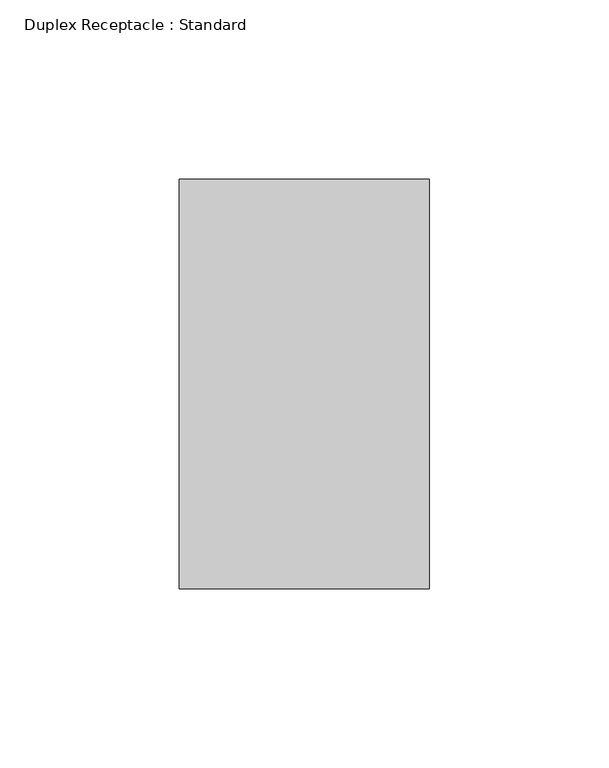
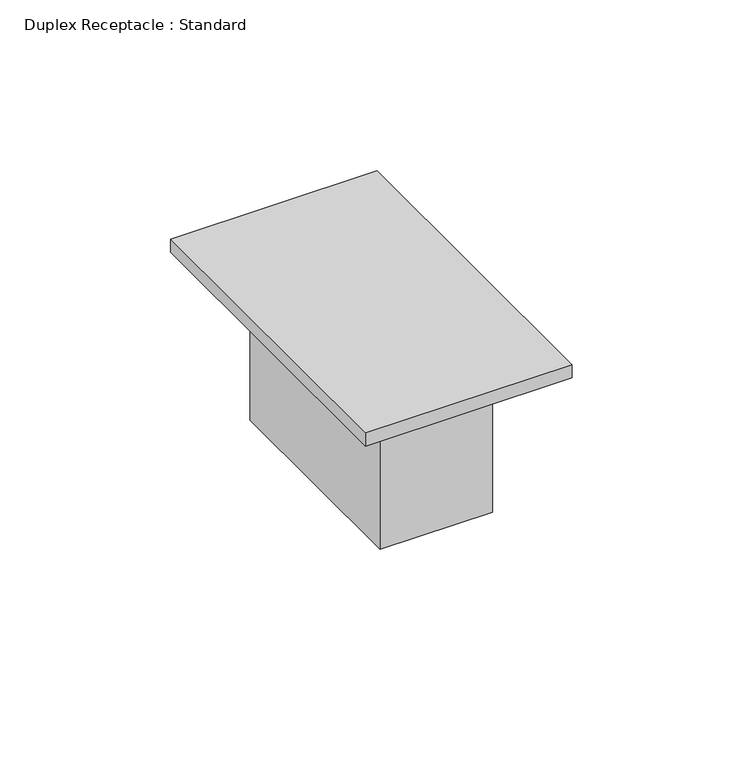
"""IFC4 building model written with IfcOpenShell, lengths in millimetres: proxy geometry, Duplex Receptacle : Standard."""

import ifcopenshell
import ifcopenshell.guid

model = None  # the IFC model being written
_history = None  # IfcOwnerHistory: only IFC2X3 demands one
_inside = {}  # id of a spatial element -> (the spatial element, [elements in it])
_under = {}  # id of a project, library or spatial element -> (it, [spatial elements below it])
_declared = {}  # id of a project -> (the project, [libraries it declares])
_typed = {}  # id of a type object -> (the type object, [elements of that type])
_made_of = {}  # id of a material, layer set ... -> (it, [elements and type objects made of it])


def new_model(schema):
    """Start an empty IFC model of exactly this schema.

    Asked for "IFC4X3", IfcOpenShell would pick the latest addendum, in which some entities
    have other attributes; the version numbers below select the first issue.
    IFC2X3 requires an IfcOwnerHistory on every rooted entity: one is made here for all.
    """
    global model, _history
    if schema == "IFC4X3":
        model = ifcopenshell.file(schema_version=(4, 3, 0, 0))
    else:
        model = ifcopenshell.file(schema=schema)
    _inside.clear()
    _under.clear()
    _declared.clear()
    _typed.clear()
    _made_of.clear()
    _history = None
    if model.schema == "IFC2X3":
        org = make("IfcOrganization", Name="unknown")
        user = make(
            "IfcPersonAndOrganization",
            ThePerson=make("IfcPerson", FamilyName="unknown"),
            TheOrganization=org,
        )
        app = make(
            "IfcApplication",
            ApplicationDeveloper=org,
            Version="unknown",
            ApplicationFullName="unknown",
            ApplicationIdentifier="unknown",
        )
        _history = make(
            "IfcOwnerHistory",
            OwningUser=user,
            OwningApplication=app,
            ChangeAction="ADDED",
            CreationDate=0,
        )
    return model


def make(cls, **values):
    """One entity of the class cls with the attributes given. An attribute that is None is left unset."""
    return model.create_entity(
        cls, **{name: value for name, value in values.items() if value is not None}
    )


def rooted(cls, **values):
    """An entity with a GlobalId (a new one), such as an element, a storey or a relation."""
    return make(cls, GlobalId=ifcopenshell.guid.new(), OwnerHistory=_history, **values)


def si_unit(unit_type, name, prefix=None):
    """IfcSIUnit, for example si_unit("LENGTHUNIT", "METRE", prefix="MILLI")."""
    return make("IfcSIUnit", UnitType=unit_type, Prefix=prefix, Name=name)


def assignment(units):
    """IfcUnitAssignment: the units of a project."""
    return None if units is None else make("IfcUnitAssignment", Units=units)


def point(xyz):
    """IfcCartesianPoint."""
    return None if xyz is None else make("IfcCartesianPoint", Coordinates=xyz)


def direction(xyz):
    """IfcDirection."""
    return None if xyz is None else make("IfcDirection", DirectionRatios=xyz)


def frame(location, z_axis=None, x_axis=None):
    """IfcAxis2Placement3D, a coordinate frame: its origin and axes. An axis left out is left unset."""
    return make(
        "IfcAxis2Placement3D",
        Location=point(location),
        Axis=direction(z_axis),
        RefDirection=direction(x_axis),
    )


def origin():
    """The frame at (0, 0, 0) with its axes left unset."""
    return frame((0.0, 0.0, 0.0))


def origin_with_axes():
    """The frame at (0, 0, 0) with the z axis (0, 0, 1) and the x axis (1, 0, 0) written out."""
    return frame((0.0, 0.0, 0.0), z_axis=(0.0, 0.0, 1.0), x_axis=(1.0, 0.0, 0.0))


def place(relative_to, where):
    """IfcLocalPlacement: puts the frame where relative to a parent placement (None: the world)."""
    return make(
        "IfcLocalPlacement", PlacementRelTo=relative_to, RelativePlacement=where
    )


def context(
    kind, dimensions, precision=None, world=None, true_north=None, identifier=None
):
    """IfcGeometricRepresentationContext, for example the 3D "Model" context."""
    return make(
        "IfcGeometricRepresentationContext",
        ContextIdentifier=identifier,
        ContextType=kind,
        CoordinateSpaceDimension=dimensions,
        Precision=precision,
        WorldCoordinateSystem=world,
        TrueNorth=true_north,
    )


def project(units=None, contexts=None):
    """IfcProject with its units and contexts."""
    return rooted(
        "IfcProject",
        Name="project",
        RepresentationContexts=contexts,
        UnitsInContext=assignment(units),
    )


def spatial(cls, under=None, at=None, **own):
    """A site, building, storey or space (cls), placed at a placement, below another one or the project."""
    s = rooted(cls, ObjectPlacement=at, **own)
    if under is not None:
        _under.setdefault(under.id(), (under, []))[1].append(s)
    return s


def polyline(points):
    """IfcPolyline through the points."""
    return make("IfcPolyline", Points=[point(p) for p in points])


def outline(outer, holes=None, kind="AREA"):
    """IfcArbitraryClosedProfileDef: a profile drawn as a closed curve; with holes, ...WithVoids."""
    if holes is None:
        return make("IfcArbitraryClosedProfileDef", ProfileType=kind, OuterCurve=outer)
    return make(
        "IfcArbitraryProfileDefWithVoids",
        ProfileType=kind,
        OuterCurve=outer,
        InnerCurves=holes,
    )


def extrude(swept, where, along, depth):
    """IfcExtrudedAreaSolid: the profile swept, set in the frame where, extruded along a direction by depth."""
    return make(
        "IfcExtrudedAreaSolid",
        SweptArea=swept,
        Position=where,
        ExtrudedDirection=direction(along),
        Depth=depth,
    )


def shape(context_of_items, identifier, shape_type, items):
    """IfcShapeRepresentation: the items that make up one representation, for example the "Body"."""
    return make(
        "IfcShapeRepresentation",
        ContextOfItems=context_of_items,
        RepresentationIdentifier=identifier,
        RepresentationType=shape_type,
        Items=items,
    )


def source(mapping_origin, context_of_items, identifier, shape_type, items):
    """IfcRepresentationMap: a shape defined once, which mapped items show again and again."""
    return make(
        "IfcRepresentationMap",
        MappingOrigin=mapping_origin,
        MappedRepresentation=shape(context_of_items, identifier, shape_type, items),
    )


def transform(
    local_origin,
    x_axis=None,
    y_axis=None,
    z_axis=None,
    scale=None,
    scale2=None,
    scale3=None,
    uniform=True,
):
    """IfcCartesianTransformationOperator3D, or its non-uniform kind. x_axis, y_axis, z_axis: its Axis1, 2, 3."""
    if uniform:
        return make(
            "IfcCartesianTransformationOperator3D",
            Axis1=direction(x_axis),
            Axis2=direction(y_axis),
            LocalOrigin=point(local_origin),
            Scale=scale,
            Axis3=direction(z_axis),
        )
    return make(
        "IfcCartesianTransformationOperator3DnonUniform",
        Axis1=direction(x_axis),
        Axis2=direction(y_axis),
        LocalOrigin=point(local_origin),
        Scale=scale,
        Axis3=direction(z_axis),
        Scale2=scale2,
        Scale3=scale3,
    )


def mapped(mapping_source, mapping_target):
    """IfcMappedItem: shows the shape of a source again, moved by a transform."""
    return make(
        "IfcMappedItem", MappingSource=mapping_source, MappingTarget=mapping_target
    )


def made_of(thing, what):
    """Note that an element or type object is made of a material, layer set ...; save() writes the relation."""
    if what is not None:
        _made_of.setdefault(what.id(), (what, []))[1].append(thing)
    return thing


def element(
    cls,
    number,
    at=None,
    inside=None,
    cuts=None,
    type_object=None,
    material=None,
    context=None,
    identifier="Body",
    shape_type=None,
    held_by="IfcProductDefinitionShape",
    body=None,
    shapes=None,
    **own,
):
    """One element of the class cls, such as IfcWall. Its Tag is "e" and its number.

    at: its placement. inside: the storey or other place that contains it. cuts: it is an
    opening in that element (IfcRelVoidsElement). A single representation is given by context,
    identifier, shape_type and body (its items); several are given by shapes. held_by: the class
    of the entity that holds the representations. save() writes the other relations.
    """
    e = rooted(cls, Tag="e%d" % number, ObjectPlacement=at, **own)
    if body is not None:
        shapes = [shape(context, identifier, shape_type, body)]
    if shapes is not None:
        e.Representation = make(held_by, Representations=shapes)
    if inside is not None:
        _inside.setdefault(inside.id(), (inside, []))[1].append(e)
    if cuts is not None:
        rooted(
            "IfcRelVoidsElement", RelatingBuildingElement=cuts, RelatedOpeningElement=e
        )
    if type_object is not None:
        _typed.setdefault(type_object.id(), (type_object, []))[1].append(e)
    return made_of(e, material)


def aggregate(whole, parts):
    """IfcRelAggregates: a whole, such as a stair, and the parts it consists of."""
    return rooted("IfcRelAggregates", RelatingObject=whole, RelatedObjects=parts)


def save(model, path):
    """Write the relations noted so far, then the file.

    IfcRelAggregates (storeys below a building ...), IfcRelContainedInSpatialStructure (elements
    in a storey), IfcRelDefinesByType, IfcRelAssociatesMaterial and IfcRelDeclares: one each for
    every whole, place, type object, material and project.
    """
    for whole, parts in _under.values():
        aggregate(whole, parts)
    for where, things in _inside.values():
        rooted(
            "IfcRelContainedInSpatialStructure",
            RelatedElements=things,
            RelatingStructure=where,
        )
    for kind, things in _typed.values():
        rooted("IfcRelDefinesByType", RelatedObjects=things, RelatingType=kind)
    for what, things in _made_of.values():
        rooted("IfcRelAssociatesMaterial", RelatedObjects=things, RelatingMaterial=what)
    for by, libraries in _declared.values():
        rooted("IfcRelDeclares", RelatingContext=by, RelatedDefinitions=libraries)
    model.write(path)


def duplex_receptacle_standard_10251bba(model_context):
    return source(origin(), model_context, "Body", "SweptSolid", [
        extrude(outline(polyline([(19.05, 38.1), (19.05, -38.1), (-19.05, -38.1), (-19.05, 38.1), (19.05, 38.1)])), frame((0.0, 0.0, -53.975), z_axis=(0.0, 0.0, 1.0), x_axis=(1.0, 0.0, 0.0)), (0.0, 0.0, 1.0), 53.975),
        extrude(outline(polyline([(34.925, 57.15), (34.925, -57.15), (-34.925, -57.15), (-34.925, 57.15), (34.925, 57.15)])), origin_with_axes(), (0.0, 0.0, 1.0), 4.7625),
    ])


if __name__ == "__main__":
    model = new_model("IFC4")
    model_context = context("Model", 3, world=origin())
    ifc_project = project(units=[si_unit("LENGTHUNIT", "METRE", prefix="MILLI")], contexts=[model_context])
    site = spatial("IfcSite", under=ifc_project)
    building = spatial("IfcBuilding", under=site)
    placement = place(None, origin())
    duplex_receptacle_standard_shape = duplex_receptacle_standard_10251bba(model_context)
    element("IfcBuildingElementProxy", 1, Name="Duplex Receptacle : Standard", ObjectType="Duplex Receptacle : Standard", at=placement, inside=building, context=model_context, shape_type="MappedRepresentation", body=[
        mapped(duplex_receptacle_standard_shape, transform((0.0, 0.0, 0.0), x_axis=(1.0, 0.0, 0.0), y_axis=(0.0, 1.0, 0.0), z_axis=(0.0, 0.0, 1.0))),
    ])
    save(model, "model.ifc")

# Revit data of these elements
# Project information
#   Project Issue Date = "Issue Date"
#   Project Status = "Project Status"
#   Client Name = "Owner"
#   Project Address = "Enter address here"
#   Project Name = "Project Name"
#   Project Number = "Project Number"
# Type "Duplex Receptacle : Standard"
#   Label = ""
#   Switch Voltage = 120 V
#   Load = 180 VA
#   Default Elevation = 1' - 6"
#   Load Classification = Receptacle
#   Assembly Code = ""
